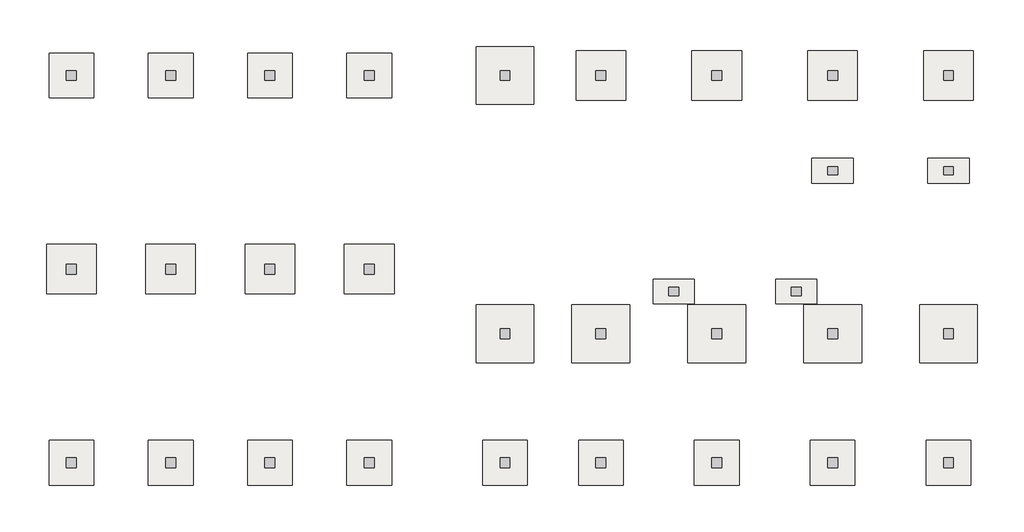
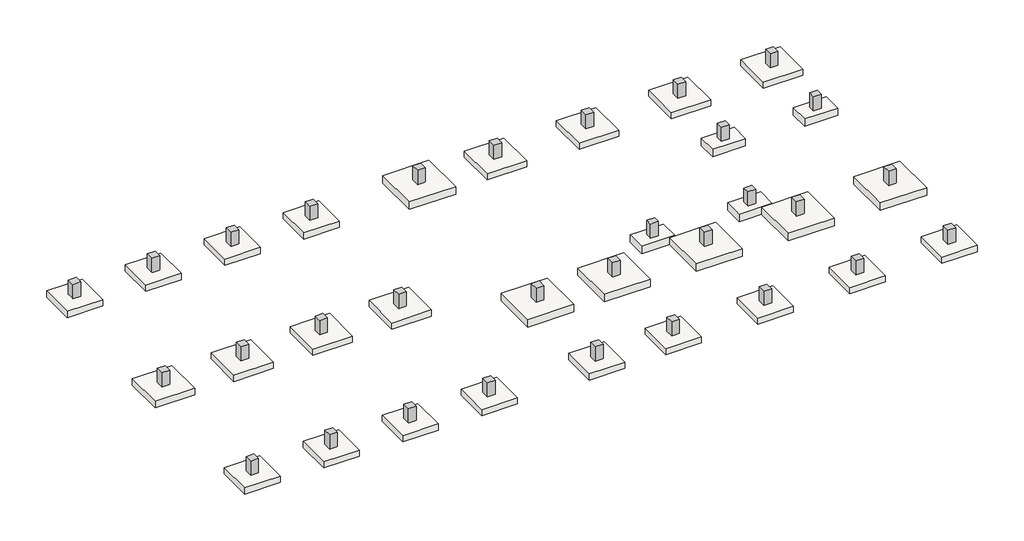
# Not in any storey: 31 columns, 31 slabs.
"""IFC4 building model written with IfcOpenShell, lengths in millimetres."""

from ifc_helpers import new_model, si_unit, frame, origin, place, context, project, spatial, polyline, outline, extrude, faceted_brep, element, save

model = new_model("IFC4")

# Units and contexts
model_context = context("Model", 3, world=origin())
ifc_project = project(units=[si_unit("LENGTHUNIT", "METRE", prefix="MILLI")], contexts=[model_context])

# Site, building
site = spatial("IfcSite", under=ifc_project)
building = spatial("IfcBuilding", under=site)

# Columns
placement = place(None, origin())
element("IfcColumn", 1, ObjectType="RC_Column_Rectangular : H_SC_AR_S15_UG PED_W600xL600_Bit_Anchor", at=placement, inside=building, context=model_context, shape_type="Brep", body=[
    faceted_brep([(300.0, 12499.5208589, -1000.0381366), (300.0, 11899.5208589, -1000.0381366), (-300.0, 11899.5208589, -1000.0381366), (-300.0, 12499.5208589, -1000.0381366), (300.0, 12499.5208589, 149.9618634), (300.0, 11899.5208589, 149.9618634), (300.0, 11899.5208589, -0.0381366), (300.0, 11899.5208589, -500.0381366), (300.0, 12499.5208589, -500.0381366), (300.0, 12499.5208589, -0.0381366), (-300.0, 11899.5208589, 149.9618634), (-300.0, 11899.5208589, -0.0381366), (-300.0, 11899.5208589, -500.0381366), (-300.0, 12499.5208589, 149.9618634), (-300.0, 12499.5208589, -0.0381366), (-300.0, 12499.5208589, -500.0381366)], [[[0, 1, 2, 3]], [[4, 5, 6, 7, 1, 0, 8, 9]], [[5, 10, 11, 12, 2, 1, 7, 6]], [[10, 13, 14, 15, 3, 2, 12, 11]], [[13, 4, 9, 8, 0, 3, 15, 14]], [[4, 13, 10, 5]]]),
])
element("IfcColumn", 2, ObjectType="RC_Column_Rectangular : H_SC_AR_S15_UG PED_W600xL600_Bit_Anchor", at=placement, inside=building, context=model_context, shape_type="SweptSolid", body=[
    extrude(outline(polyline([(6300.0, 12499.5208589), (6300.0, 11899.5208589), (5700.0, 11899.5208589), (5700.0, 12499.5208589), (6300.0, 12499.5208589)])), frame((0.0, 0.0, -1000.0381366), z_axis=(0.0, 0.0, 1.0), x_axis=(1.0, 0.0, 0.0)), (0.0, 0.0, 1.0), 1150.0),
])
element("IfcColumn", 3, ObjectType="RC_Column_Rectangular : H_SC_AR_S15_UG PED_W600xL600_Bit_Anchor", at=placement, inside=building, context=model_context, shape_type="SweptSolid", body=[
    extrude(outline(polyline([(12300.0, 12499.5208589), (12300.0, 11899.5208589), (11700.0, 11899.5208589), (11700.0, 12499.5208589), (12300.0, 12499.5208589)])), frame((0.0, 0.0, -1000.0381366), z_axis=(0.0, 0.0, 1.0), x_axis=(1.0, 0.0, 0.0)), (0.0, 0.0, 1.0), 1150.0),
])
element("IfcColumn", 4, ObjectType="RC_Column_Rectangular : H_SC_AR_S15_UG PED_W600xL600_Bit_Anchor", at=placement, inside=building, context=model_context, shape_type="SweptSolid", body=[
    extrude(outline(polyline([(18300.0, 12499.5208589), (18300.0, 11899.5208589), (17700.0, 11899.5208589), (17700.0, 12499.5208589), (18300.0, 12499.5208589)])), frame((0.0, 0.0, -1000.0381366), z_axis=(0.0, 0.0, 1.0), x_axis=(1.0, 0.0, 0.0)), (0.0, 0.0, 1.0), 1150.0),
])
element("IfcColumn", 5, ObjectType="RC_Column_Rectangular : H_SC_AR_S15_UG PED_W600xL600_Bit_Anchor", at=placement, inside=building, context=model_context, shape_type="Brep", body=[
    faceted_brep([(300.0, 24199.5208589, -1000.0381366), (300.0, 23599.5208589, -1000.0381366), (-300.0, 23599.5208589, -1000.0381366), (-300.0, 24199.5208589, -1000.0381366), (300.0, 24199.5208589, 149.9618634), (300.0, 23599.5208589, 149.9618634), (300.0, 23599.5208589, -0.0381366), (300.0, 23599.5208589, -500.0381366), (300.0, 24199.5208589, -500.0381366), (300.0, 24199.5208589, -0.0381366), (-300.0, 23599.5208589, 149.9618634), (-300.0, 23599.5208589, -0.0381366), (-300.0, 23599.5208589, -500.0381366), (-300.0, 24199.5208589, 149.9618634)], [[[0, 1, 2, 3]], [[4, 5, 6, 7, 1, 0, 8, 9]], [[5, 10, 11, 12, 2, 1, 7, 6]], [[10, 13, 3, 2, 12, 11]], [[13, 4, 9, 8, 0, 3]], [[4, 13, 10, 5]]]),
])
element("IfcColumn", 6, ObjectType="RC_Column_Rectangular : H_SC_AR_S15_UG PED_W600xL600_Bit_Anchor", at=placement, inside=building, context=model_context, shape_type="Brep", body=[
    faceted_brep([(6300.0, 24199.5208589, -1000.0381366), (6300.0, 23599.5208589, -1000.0381366), (5700.0, 23599.5208589, -1000.0381366), (5700.0, 24199.5208589, -1000.0381366), (6300.0, 24199.5208589, 149.9618634), (6300.0, 23599.5208589, 149.9618634), (6300.0, 23599.5208589, -0.0381366), (6300.0, 23599.5208589, -500.0381366), (6300.0, 24199.5208589, -500.0381366), (6300.0, 24199.5208589, -0.0381366), (5700.0, 23599.5208589, 149.9618634), (5700.0, 23599.5208589, -0.0381366), (5700.0, 23599.5208589, -500.0381366), (5700.0, 24199.5208589, 149.9618634), (5700.0, 24199.5208589, -0.0381366), (5700.0, 24199.5208589, -500.0381366)], [[[0, 1, 2, 3]], [[4, 5, 6, 7, 1, 0, 8, 9]], [[5, 10, 11, 12, 2, 1, 7, 6]], [[10, 13, 14, 15, 3, 2, 12, 11]], [[13, 4, 9, 8, 0, 3, 15, 14]], [[4, 13, 10, 5]]]),
])
element("IfcColumn", 7, ObjectType="RC_Column_Rectangular : H_SC_AR_S15_UG PED_W600xL600_Bit_Anchor", at=placement, inside=building, context=model_context, shape_type="Brep", body=[
    faceted_brep([(12300.0, 24199.5208589, -1000.0381366), (12300.0, 23599.5208589, -1000.0381366), (11700.0, 23599.5208589, -1000.0381366), (11700.0, 24199.5208589, -1000.0381366), (12300.0, 24199.5208589, 149.9618634), (12300.0, 23599.5208589, 149.9618634), (12300.0, 23599.5208589, -0.0381366), (12300.0, 23599.5208589, -500.0381366), (12300.0, 24199.5208589, -500.0381366), (12300.0, 24199.5208589, -0.0381366), (11700.0, 23599.5208589, 149.9618634), (11700.0, 23599.5208589, -0.0381366), (11700.0, 23599.5208589, -500.0381366), (11700.0, 24199.5208589, 149.9618634), (11700.0, 24199.5208589, -0.0381366), (11700.0, 24199.5208589, -500.0381366)], [[[0, 1, 2, 3]], [[4, 5, 6, 7, 1, 0, 8, 9]], [[5, 10, 11, 12, 2, 1, 7, 6]], [[10, 13, 14, 15, 3, 2, 12, 11]], [[13, 4, 9, 8, 0, 3, 15, 14]], [[4, 13, 10, 5]]]),
])
element("IfcColumn", 8, ObjectType="RC_Column_Rectangular : H_SC_AR_S15_UG PED_W600xL600_Bit_Anchor", at=placement, inside=building, context=model_context, shape_type="Brep", body=[
    faceted_brep([(18300.0, 24199.5208589, -1000.0381366), (18300.0, 23599.5208589, -1000.0381366), (17700.0, 23599.5208589, -1000.0381366), (17700.0, 24199.5208589, -1000.0381366), (18300.0, 24199.5208589, 149.9618634), (18300.0, 23599.5208589, 149.9618634), (18300.0, 23599.5208589, -0.0381366), (18300.0, 23599.5208589, -500.0381366), (18300.0, 24199.5208589, -500.0381366), (18300.0, 24199.5208589, -0.0381366), (17700.0, 23599.5208589, 149.9618634), (17700.0, 23599.5208589, -0.0381366), (17700.0, 23599.5208589, -500.0381366), (17700.0, 24199.5208589, 149.9618634), (17700.0, 24199.5208589, -0.0381366), (17700.0, 24199.5208589, -500.0381366)], [[[0, 1, 2, 3]], [[4, 5, 6, 7, 1, 0, 8, 9]], [[5, 10, 11, 12, 2, 1, 7, 6]], [[10, 13, 14, 15, 3, 2, 12, 11]], [[13, 4, 9, 8, 0, 3, 15, 14]], [[4, 13, 10, 5]]]),
])
element("IfcColumn", 9, ObjectType="RC_Column_Rectangular : H_SC_AR_S15_UG PED_W600xL600_Bit_Anchor", at=placement, inside=building, context=model_context, shape_type="Brep", body=[
    faceted_brep([(26500.0, 24199.5208589, -1000.0381366), (26500.0, 23599.5208589, -1000.0381366), (25900.0, 23599.5208589, -1000.0381366), (25900.0, 24199.5208589, -1000.0381366), (26500.0, 24199.5208589, 149.9618634), (26500.0, 23599.5208589, 149.9618634), (26500.0, 23599.5208589, -0.0381366), (26500.0, 23599.5208589, -500.0381366), (26500.0, 24199.5208589, -500.0381366), (26500.0, 24199.5208589, -0.0381366), (25900.0, 23599.5208589, 149.9618634), (25900.0, 23599.5208589, -0.0381366), (25900.0, 23599.5208589, -500.0381366), (25900.0, 24199.5208589, 149.9618634), (25900.0, 24199.5208589, -0.0381366), (25900.0, 24199.5208589, -500.0381366)], [[[0, 1, 2, 3]], [[4, 5, 6, 7, 1, 0, 8, 9]], [[5, 10, 11, 12, 2, 1, 7, 6]], [[10, 13, 14, 15, 3, 2, 12, 11]], [[13, 4, 9, 8, 0, 3, 15, 14]], [[4, 13, 10, 5]]]),
])
element("IfcColumn", 10, ObjectType="RC_Column_Rectangular : H_SC_AR_S15_UG PED_W600xL600_Bit_Anchor", at=placement, inside=building, context=model_context, shape_type="Brep", body=[
    faceted_brep([(32300.0, 24199.5208589, -1000.0381366), (32300.0, 23599.5208589, -1000.0381366), (31700.0, 23599.5208589, -1000.0381366), (31700.0, 24199.5208589, -1000.0381366), (32300.0, 24199.5208589, 149.9618634), (32300.0, 23599.5208589, 149.9618634), (32300.0, 23599.5208589, -0.0381366), (32300.0, 23599.5208589, -500.0381366), (32300.0, 24199.5208589, -500.0381366), (32300.0, 24199.5208589, -0.0381366), (31700.0, 23599.5208589, 149.9618634), (31700.0, 23599.5208589, -0.0381366), (31700.0, 23599.5208589, -500.0381366), (31700.0, 24199.5208589, 149.9618634), (31700.0, 24199.5208589, -0.0381366), (31700.0, 24199.5208589, -500.0381366)], [[[0, 1, 2, 3]], [[4, 5, 6, 7, 1, 0, 8, 9]], [[5, 10, 11, 12, 2, 1, 7, 6]], [[10, 13, 14, 15, 3, 2, 12, 11]], [[13, 4, 9, 8, 0, 3, 15, 14]], [[4, 13, 10, 5]]]),
])
element("IfcColumn", 11, ObjectType="RC_Column_Rectangular : H_SC_AR_S15_UG PED_W600xL600_Bit_Anchor", at=placement, inside=building, context=model_context, shape_type="Brep", body=[
    faceted_brep([(39300.0, 24199.5208589, -1000.0381366), (39300.0, 23599.5208589, -1000.0381366), (38700.0, 23599.5208589, -1000.0381366), (38700.0, 24199.5208589, -1000.0381366), (39300.0, 24199.5208589, 149.9618634), (39300.0, 23599.5208589, 149.9618634), (39300.0, 23599.5208589, -0.0381366), (39300.0, 23599.5208589, -500.0381366), (39300.0, 24199.5208589, -500.0381366), (39300.0, 24199.5208589, -0.0381366), (38700.0, 23599.5208589, 149.9618634), (38700.0, 23599.5208589, -0.0381366), (38700.0, 23599.5208589, -500.0381366), (38700.0, 24199.5208589, 149.9618634), (38700.0, 24199.5208589, -0.0381366), (38700.0, 24199.5208589, -500.0381366)], [[[0, 1, 2, 3]], [[4, 5, 6, 7, 1, 0, 8, 9]], [[5, 10, 11, 12, 2, 1, 7, 6]], [[10, 13, 14, 15, 3, 2, 12, 11]], [[13, 4, 9, 8, 0, 3, 15, 14]], [[4, 13, 10, 5]]]),
])
element("IfcColumn", 12, ObjectType="RC_Column_Rectangular : H_SC_AR_S15_UG PED_W600xL600_Bit_Anchor", at=placement, inside=building, context=model_context, shape_type="Brep", body=[
    faceted_brep([(46300.0, 24199.5208589, -1000.0381366), (46300.0, 23599.5208589, -1000.0381366), (45700.0, 23599.5208589, -1000.0381366), (45700.0, 24199.5208589, -1000.0381366), (46300.0, 24199.5208589, 149.9618634), (46300.0, 23599.5208589, 149.9618634), (46300.0, 23599.5208589, -0.0381366), (46300.0, 23599.5208589, -500.0381366), (46300.0, 24199.5208589, -500.0381366), (46300.0, 24199.5208589, -0.0381366), (45700.0, 23599.5208589, 149.9618634), (45700.0, 23599.5208589, -0.0381366), (45700.0, 23599.5208589, -500.0381366), (45700.0, 24199.5208589, 149.9618634), (45700.0, 24199.5208589, -0.0381366), (45700.0, 24199.5208589, -500.0381366)], [[[0, 1, 2, 3]], [[4, 5, 6, 7, 1, 0, 8, 9]], [[5, 10, 11, 12, 2, 1, 7, 6]], [[10, 13, 14, 15, 3, 2, 12, 11]], [[13, 4, 9, 8, 0, 3, 15, 14]], [[4, 13, 10, 5]]]),
])
element("IfcColumn", 13, ObjectType="RC_Column_Rectangular : H_SC_AR_S15_UG PED_W600xL600_Bit_Anchor", at=placement, inside=building, context=model_context, shape_type="Brep", body=[
    faceted_brep([(53300.0, 24199.5208589, -1000.0381366), (53300.0, 23599.5208589, -1000.0381366), (52700.0, 23599.5208589, -1000.0381366), (52700.0, 24199.5208589, -1000.0381366), (53300.0, 24199.5208589, 149.9618634), (53300.0, 23599.5208589, 149.9618634), (53300.0, 23599.5208589, -0.0381366), (53300.0, 23599.5208589, -500.0381366), (52700.0, 23599.5208589, 149.9618634), (52700.0, 23599.5208589, -0.0381366), (52700.0, 23599.5208589, -500.0381366), (52700.0, 24199.5208589, 149.9618634), (52700.0, 24199.5208589, -0.0381366), (52700.0, 24199.5208589, -500.0381366)], [[[0, 1, 2, 3]], [[4, 5, 6, 7, 1, 0]], [[5, 8, 9, 10, 2, 1, 7, 6]], [[8, 11, 12, 13, 3, 2, 10, 9]], [[11, 4, 0, 3, 13, 12]], [[4, 11, 8, 5]]]),
])
element("IfcColumn", 14, ObjectType="RC_Column_Rectangular : H_SC_AR_S15_UG PED_W600xL600_Bit_Anchor", at=placement, inside=building, context=model_context, shape_type="SweptSolid", body=[
    extrude(outline(polyline([(26500.0, 8599.5208589), (26500.0, 7999.5208589), (25900.0, 7999.5208589), (25900.0, 8599.5208589), (26500.0, 8599.5208589)])), frame((0.0, 0.0, -1000.0381366), z_axis=(0.0, 0.0, 1.0), x_axis=(1.0, 0.0, 0.0)), (0.0, 0.0, 1.0), 1150.0),
])
element("IfcColumn", 15, ObjectType="RC_Column_Rectangular : H_SC_AR_S15_UG PED_W600xL600_Bit_Anchor", at=placement, inside=building, context=model_context, shape_type="SweptSolid", body=[
    extrude(outline(polyline([(32300.0, 8599.5208589), (32300.0, 7999.5208589), (31700.0, 7999.5208589), (31700.0, 8599.5208589), (32300.0, 8599.5208589)])), frame((0.0, 0.0, -1000.0381366), z_axis=(0.0, 0.0, 1.0), x_axis=(1.0, 0.0, 0.0)), (0.0, 0.0, 1.0), 1150.0),
])
element("IfcColumn", 16, ObjectType="RC_Column_Rectangular : H_SC_AR_S15_UG PED_W600xL600_Bit_Anchor", at=placement, inside=building, context=model_context, shape_type="SweptSolid", body=[
    extrude(outline(polyline([(39300.0, 8599.5208589), (39300.0, 7999.5208589), (38700.0, 7999.5208589), (38700.0, 8599.5208589), (39300.0, 8599.5208589)])), frame((0.0, 0.0, -1000.0381366), z_axis=(0.0, 0.0, 1.0), x_axis=(1.0, 0.0, 0.0)), (0.0, 0.0, 1.0), 1150.0),
])
element("IfcColumn", 17, ObjectType="RC_Column_Rectangular : H_SC_AR_S15_UG PED_W600xL600_Bit_Anchor", at=placement, inside=building, context=model_context, shape_type="SweptSolid", body=[
    extrude(outline(polyline([(46300.0, 8599.5208589), (46300.0, 7999.5208589), (45700.0, 7999.5208589), (45700.0, 8599.5208589), (46300.0, 8599.5208589)])), frame((0.0, 0.0, -1000.0381366), z_axis=(0.0, 0.0, 1.0), x_axis=(1.0, 0.0, 0.0)), (0.0, 0.0, 1.0), 1150.0),
])
element("IfcColumn", 18, ObjectType="RC_Column_Rectangular : H_SC_AR_S15_UG PED_W600xL600_Bit_Anchor", at=placement, inside=building, context=model_context, shape_type="Brep", body=[
    faceted_brep([(53300.0, 8599.5208589, -1000.0381366), (53300.0, 7999.5208589, -1000.0381366), (52700.0, 7999.5208589, -1000.0381366), (52700.0, 8599.5208589, -1000.0381366), (53300.0, 8599.5208589, 149.9618634), (53300.0, 7999.5208589, 149.9618634), (53300.0, 7999.5208589, -0.0381366), (53300.0, 7999.5208589, -500.0381366), (53300.0, 8599.5208589, -500.0381366), (53300.0, 8599.5208589, -0.0381366), (52700.0, 7999.5208589, 149.9618634), (52700.0, 7999.5208589, -0.0381366), (52700.0, 7999.5208589, -500.0381366), (52700.0, 8599.5208589, 149.9618634), (52700.0, 8599.5208589, -0.0381366), (52700.0, 8599.5208589, -500.0381366)], [[[0, 1, 2, 3]], [[4, 5, 6, 7, 1, 0, 8, 9]], [[5, 10, 11, 12, 2, 1, 7, 6]], [[10, 13, 14, 15, 3, 2, 12, 11]], [[13, 4, 9, 8, 0, 3, 15, 14]], [[4, 13, 10, 5]]]),
])
element("IfcColumn", 19, ObjectType="RC_Column_Rectangular : H_SC_AR_S15_UG PED_W600xL600_Bit_Anchor", at=placement, inside=building, context=model_context, shape_type="Brep", body=[
    faceted_brep([(300.0, 799.5208589, -1000.0381366), (300.0, 199.5208589, -1000.0381366), (-300.0, 199.5208589, -1000.0381366), (-300.0, 799.5208589, -1000.0381366), (300.0, 799.5208589, 149.9618634), (300.0, 199.5208589, 149.9618634), (300.0, 199.5208589, -0.0381366), (300.0, 199.5208589, -500.0381366), (300.0, 799.5208589, -500.0381366), (300.0, 799.5208589, -0.0381366), (-300.0, 199.5208589, 149.9618634), (-300.0, 799.5208589, 149.9618634), (-300.0, 799.5208589, -0.0381366), (-300.0, 799.5208589, -500.0381366)], [[[0, 1, 2, 3]], [[4, 5, 6, 7, 1, 0, 8, 9]], [[5, 10, 2, 1, 7, 6]], [[10, 11, 12, 13, 3, 2]], [[11, 4, 9, 8, 0, 3, 13, 12]], [[4, 11, 10, 5]]]),
])
element("IfcColumn", 20, ObjectType="RC_Column_Rectangular : H_SC_AR_S15_UG PED_W600xL600_Bit_Anchor", at=placement, inside=building, context=model_context, shape_type="Brep", body=[
    faceted_brep([(6300.0, 799.5208589, -1000.0381366), (6300.0, 199.5208589, -1000.0381366), (5700.0, 199.5208589, -1000.0381366), (5700.0, 799.5208589, -1000.0381366), (6300.0, 799.5208589, 149.9618634), (6300.0, 199.5208589, 149.9618634), (6300.0, 199.5208589, -0.0381366), (6300.0, 199.5208589, -500.0381366), (6300.0, 799.5208589, -500.0381366), (6300.0, 799.5208589, -0.0381366), (5700.0, 199.5208589, 149.9618634), (5700.0, 199.5208589, -0.0381366), (5700.0, 199.5208589, -500.0381366), (5700.0, 799.5208589, 149.9618634), (5700.0, 799.5208589, -0.0381366), (5700.0, 799.5208589, -500.0381366)], [[[0, 1, 2, 3]], [[4, 5, 6, 7, 1, 0, 8, 9]], [[5, 10, 11, 12, 2, 1, 7, 6]], [[10, 13, 14, 15, 3, 2, 12, 11]], [[13, 4, 9, 8, 0, 3, 15, 14]], [[4, 13, 10, 5]]]),
])
element("IfcColumn", 21, ObjectType="RC_Column_Rectangular : H_SC_AR_S15_UG PED_W600xL600_Bit_Anchor", at=placement, inside=building, context=model_context, shape_type="Brep", body=[
    faceted_brep([(12300.0, 799.5208589, -1000.0381366), (12300.0, 199.5208589, -1000.0381366), (11700.0, 199.5208589, -1000.0381366), (11700.0, 799.5208589, -1000.0381366), (12300.0, 799.5208589, 149.9618634), (12300.0, 199.5208589, 149.9618634), (12300.0, 199.5208589, -0.0381366), (12300.0, 199.5208589, -500.0381366), (12300.0, 799.5208589, -500.0381366), (12300.0, 799.5208589, -0.0381366), (11700.0, 199.5208589, 149.9618634), (11700.0, 199.5208589, -0.0381366), (11700.0, 199.5208589, -500.0381366), (11700.0, 799.5208589, 149.9618634), (11700.0, 799.5208589, -0.0381366), (11700.0, 799.5208589, -500.0381366)], [[[0, 1, 2, 3]], [[4, 5, 6, 7, 1, 0, 8, 9]], [[5, 10, 11, 12, 2, 1, 7, 6]], [[10, 13, 14, 15, 3, 2, 12, 11]], [[13, 4, 9, 8, 0, 3, 15, 14]], [[4, 13, 10, 5]]]),
])
element("IfcColumn", 22, ObjectType="RC_Column_Rectangular : H_SC_AR_S15_UG PED_W600xL600_Bit_Anchor", at=placement, inside=building, context=model_context, shape_type="Brep", body=[
    faceted_brep([(18300.0, 799.5208589, -1000.0381366), (18300.0, 199.5208589, -1000.0381366), (17700.0, 199.5208589, -1000.0381366), (17700.0, 799.5208589, -1000.0381366), (18300.0, 799.5208589, 149.9618634), (18300.0, 199.5208589, 149.9618634), (18300.0, 199.5208589, -0.0381366), (18300.0, 199.5208589, -500.0381366), (18300.0, 799.5208589, -500.0381366), (18300.0, 799.5208589, -0.0381366), (17700.0, 199.5208589, 149.9618634), (17700.0, 199.5208589, -0.0381366), (17700.0, 199.5208589, -500.0381366), (17700.0, 799.5208589, 149.9618634), (17700.0, 799.5208589, -0.0381366), (17700.0, 799.5208589, -500.0381366)], [[[0, 1, 2, 3]], [[4, 5, 6, 7, 1, 0, 8, 9]], [[5, 10, 11, 12, 2, 1, 7, 6]], [[10, 13, 14, 15, 3, 2, 12, 11]], [[13, 4, 9, 8, 0, 3, 15, 14]], [[4, 13, 10, 5]]]),
])
element("IfcColumn", 23, ObjectType="RC_Column_Rectangular : H_SC_AR_S15_UG PED_W600xL600_Bit_Anchor", at=placement, inside=building, context=model_context, shape_type="Brep", body=[
    faceted_brep([(26500.0, 799.5208589, -1000.0381366), (26500.0, 199.5208589, -1000.0381366), (25900.0, 199.5208589, -1000.0381366), (25900.0, 799.5208589, -1000.0381366), (26500.0, 799.5208589, 149.9618634), (26500.0, 199.5208589, 149.9618634), (26500.0, 199.5208589, -0.0381366), (26500.0, 199.5208589, -500.0381366), (26500.0, 799.5208589, -500.0381366), (26500.0, 799.5208589, -0.0381366), (25900.0, 199.5208589, 149.9618634), (25900.0, 199.5208589, -0.0381366), (25900.0, 199.5208589, -500.0381366), (25900.0, 799.5208589, 149.9618634), (25900.0, 799.5208589, -0.0381366), (25900.0, 799.5208589, -500.0381366)], [[[0, 1, 2, 3]], [[4, 5, 6, 7, 1, 0, 8, 9]], [[5, 10, 11, 12, 2, 1, 7, 6]], [[10, 13, 14, 15, 3, 2, 12, 11]], [[13, 4, 9, 8, 0, 3, 15, 14]], [[4, 13, 10, 5]]]),
])
element("IfcColumn", 24, ObjectType="RC_Column_Rectangular : H_SC_AR_S15_UG PED_W600xL600_Bit_Anchor", at=placement, inside=building, context=model_context, shape_type="Brep", body=[
    faceted_brep([(32300.0, 799.5208589, -1000.0381366), (32300.0, 199.5208589, -1000.0381366), (31700.0, 199.5208589, -1000.0381366), (31700.0, 799.5208589, -1000.0381366), (32300.0, 799.5208589, 149.9618634), (32300.0, 199.5208589, 149.9618634), (32300.0, 199.5208589, -0.0381366), (32300.0, 199.5208589, -500.0381366), (32300.0, 799.5208589, -500.0381366), (32300.0, 799.5208589, -0.0381366), (31700.0, 199.5208589, 149.9618634), (31700.0, 199.5208589, -0.0381366), (31700.0, 199.5208589, -500.0381366), (31700.0, 799.5208589, 149.9618634), (31700.0, 799.5208589, -0.0381366), (31700.0, 799.5208589, -500.0381366)], [[[0, 1, 2, 3]], [[4, 5, 6, 7, 1, 0, 8, 9]], [[5, 10, 11, 12, 2, 1, 7, 6]], [[10, 13, 14, 15, 3, 2, 12, 11]], [[13, 4, 9, 8, 0, 3, 15, 14]], [[4, 13, 10, 5]]]),
])
element("IfcColumn", 25, ObjectType="RC_Column_Rectangular : H_SC_AR_S15_UG PED_W600xL600_Bit_Anchor", at=placement, inside=building, context=model_context, shape_type="Brep", body=[
    faceted_brep([(39300.0, 799.5208589, -1000.0381366), (39300.0, 199.5208589, -1000.0381366), (38700.0, 199.5208589, -1000.0381366), (38700.0, 799.5208589, -1000.0381366), (39300.0, 799.5208589, 149.9618634), (39300.0, 199.5208589, 149.9618634), (39300.0, 199.5208589, -0.0381366), (39300.0, 199.5208589, -500.0381366), (39300.0, 799.5208589, -500.0381366), (39300.0, 799.5208589, -0.0381366), (38700.0, 199.5208589, 149.9618634), (38700.0, 199.5208589, -0.0381366), (38700.0, 199.5208589, -500.0381366), (38700.0, 799.5208589, 149.9618634), (38700.0, 799.5208589, -0.0381366), (38700.0, 799.5208589, -500.0381366)], [[[0, 1, 2, 3]], [[4, 5, 6, 7, 1, 0, 8, 9]], [[5, 10, 11, 12, 2, 1, 7, 6]], [[10, 13, 14, 15, 3, 2, 12, 11]], [[13, 4, 9, 8, 0, 3, 15, 14]], [[4, 13, 10, 5]]]),
])
element("IfcColumn", 26, ObjectType="RC_Column_Rectangular : H_SC_AR_S15_UG PED_W600xL600_Bit_Anchor", at=placement, inside=building, context=model_context, shape_type="Brep", body=[
    faceted_brep([(46300.0, 799.5208589, -1000.0381366), (46300.0, 199.5208589, -1000.0381366), (45700.0, 199.5208589, -1000.0381366), (45700.0, 799.5208589, -1000.0381366), (46300.0, 799.5208589, 149.9618634), (46300.0, 199.5208589, 149.9618634), (46300.0, 199.5208589, -0.0381366), (46300.0, 199.5208589, -500.0381366), (46300.0, 799.5208589, -500.0381366), (46300.0, 799.5208589, -0.0381366), (45700.0, 199.5208589, 149.9618634), (45700.0, 199.5208589, -0.0381366), (45700.0, 199.5208589, -500.0381366), (45700.0, 799.5208589, 149.9618634), (45700.0, 799.5208589, -0.0381366), (45700.0, 799.5208589, -500.0381366)], [[[0, 1, 2, 3]], [[4, 5, 6, 7, 1, 0, 8, 9]], [[5, 10, 11, 12, 2, 1, 7, 6]], [[10, 13, 14, 15, 3, 2, 12, 11]], [[13, 4, 9, 8, 0, 3, 15, 14]], [[4, 13, 10, 5]]]),
])
element("IfcColumn", 27, ObjectType="RC_Column_Rectangular : H_SC_AR_S15_UG PED_W600xL600_Bit_Anchor", at=placement, inside=building, context=model_context, shape_type="Brep", body=[
    faceted_brep([(53300.0, 799.5208589, -1000.0381366), (53300.0, 199.5208589, -1000.0381366), (52700.0, 199.5208589, -1000.0381366), (52700.0, 799.5208589, -1000.0381366), (53300.0, 799.5208589, 149.9618634), (53300.0, 199.5208589, 149.9618634), (53300.0, 799.5208589, -500.0381366), (53300.0, 799.5208589, -0.0381366), (52700.0, 199.5208589, 149.9618634), (52700.0, 199.5208589, -0.0381366), (52700.0, 199.5208589, -500.0381366), (52700.0, 799.5208589, 149.9618634), (52700.0, 799.5208589, -0.0381366), (52700.0, 799.5208589, -500.0381366)], [[[0, 1, 2, 3]], [[4, 5, 1, 0, 6, 7]], [[5, 8, 9, 10, 2, 1]], [[8, 11, 12, 13, 3, 2, 10, 9]], [[11, 4, 7, 6, 0, 3, 13, 12]], [[4, 11, 8, 5]]]),
])
element("IfcColumn", 28, ObjectType="RC_Column_Rectangular : H_SC_AR_S15_UG PED_W600xL500_Bit_PD1A", at=placement, inside=building, context=model_context, shape_type="Brep", body=[
    faceted_brep([(52700.0, 18399.5208589, -1000.0381366), (53300.0, 18399.5208589, -1000.0381366), (53300.0, 17899.5208589, -1000.0381366), (52700.0, 17899.5208589, -1000.0381366), (52700.0, 18399.5208589, 149.9618634), (53300.0, 18399.5208589, 149.9618634), (53300.0, 18399.5208589, -0.0381366), (53300.0, 18399.5208589, -500.0381366), (52700.0, 18399.5208589, -500.0381366), (52700.0, 18399.5208589, -0.0381366), (53300.0, 17899.5208589, 149.9618634), (53300.0, 17899.5208589, -0.0381366), (53300.0, 17899.5208589, -500.0381366), (52700.0, 17899.5208589, 149.9618634), (52700.0, 17899.5208589, -0.0381366), (52700.0, 17899.5208589, -500.0381366)], [[[0, 1, 2, 3]], [[4, 5, 6, 7, 1, 0, 8, 9]], [[5, 10, 11, 12, 2, 1, 7, 6]], [[10, 13, 14, 15, 3, 2, 12, 11]], [[13, 4, 9, 8, 0, 3, 15, 14]], [[4, 13, 10, 5]]]),
])
element("IfcColumn", 29, ObjectType="RC_Column_Rectangular : H_SC_AR_S15_UG PED_W600xL500_Bit_PD1A", at=placement, inside=building, context=model_context, shape_type="SweptSolid", body=[
    extrude(outline(polyline([(45700.0, 18399.5208589), (46300.0, 18399.5208589), (46300.0, 17899.5208589), (45700.0, 17899.5208589), (45700.0, 18399.5208589)])), frame((0.0, 0.0, -1000.0381366), z_axis=(0.0, 0.0, 1.0), x_axis=(1.0, 0.0, 0.0)), (0.0, 0.0, 1.0), 1150.0),
])
element("IfcColumn", 30, ObjectType="RC_Column_Rectangular : H_SC_AR_S15_UG PED_W600xL500_Bit_PD1A", at=placement, inside=building, context=model_context, shape_type="SweptSolid", body=[
    extrude(outline(polyline([(36100.0, 11099.5208589), (36700.0, 11099.5208589), (36700.0, 10599.5208589), (36100.0, 10599.5208589), (36100.0, 11099.5208589)])), frame((0.0, 0.0, -1000.0381366), z_axis=(0.0, 0.0, 1.0), x_axis=(1.0, 0.0, 0.0)), (0.0, 0.0, 1.0), 1150.0),
])
element("IfcColumn", 31, ObjectType="RC_Column_Rectangular : H_SC_AR_S15_UG PED_W600xL500_Bit_PD1A", at=placement, inside=building, context=model_context, shape_type="SweptSolid", body=[
    extrude(outline(polyline([(43500.0, 11099.5208589), (44100.0, 11099.5208589), (44100.0, 10599.5208589), (43500.0, 10599.5208589), (43500.0, 11099.5208589)])), frame((0.0, 0.0, -1000.0381366), z_axis=(0.0, 0.0, 1.0), x_axis=(1.0, 0.0, 0.0)), (0.0, 0.0, 1.0), 1150.0),
])

# Slabs
element("IfcSlab", 32, ObjectType="Foundation Rectangular (Non-Pile) : H_SF_AR_S18_W3000xL3000xT500_Bitumen_F2", at=placement, inside=building, context=model_context, shape_type="SweptSolid", body=[
    extrude(outline(polyline([(1500.0, 13699.5208589), (1500.0, 10699.5208589), (-1500.0, 10699.5208589), (-1500.0, 13699.5208589), (1500.0, 13699.5208589)])), frame((0.0, 0.0, -1500.0381366), z_axis=(0.0, 0.0, 1.0), x_axis=(1.0, 0.0, 0.0)), (0.0, 0.0, 1.0), 500.0),
])
element("IfcSlab", 33, ObjectType="Foundation Rectangular (Non-Pile) : H_SF_AR_S18_W3000xL3000xT500_Bitumen_F2", at=placement, inside=building, context=model_context, shape_type="SweptSolid", body=[
    extrude(outline(polyline([(7500.0, 13699.5208589), (7500.0, 10699.5208589), (4500.0, 10699.5208589), (4500.0, 13699.5208589), (7500.0, 13699.5208589)])), frame((0.0, 0.0, -1500.0381366), z_axis=(0.0, 0.0, 1.0), x_axis=(1.0, 0.0, 0.0)), (0.0, 0.0, 1.0), 500.0),
])
element("IfcSlab", 34, ObjectType="Foundation Rectangular (Non-Pile) : H_SF_AR_S18_W3000xL3000xT500_Bitumen_F2", at=placement, inside=building, context=model_context, shape_type="SweptSolid", body=[
    extrude(outline(polyline([(13500.0, 13699.5208589), (13500.0, 10699.5208589), (10500.0, 10699.5208589), (10500.0, 13699.5208589), (13500.0, 13699.5208589)])), frame((0.0, 0.0, -1500.0381366), z_axis=(0.0, 0.0, 1.0), x_axis=(1.0, 0.0, 0.0)), (0.0, 0.0, 1.0), 500.0),
])
element("IfcSlab", 35, ObjectType="Foundation Rectangular (Non-Pile) : H_SF_AR_S18_W3000xL3000xT500_Bitumen_F2", at=placement, inside=building, context=model_context, shape_type="SweptSolid", body=[
    extrude(outline(polyline([(19500.0, 13699.5208589), (19500.0, 10699.5208589), (16500.0, 10699.5208589), (16500.0, 13699.5208589), (19500.0, 13699.5208589)])), frame((0.0, 0.0, -1500.0381366), z_axis=(0.0, 0.0, 1.0), x_axis=(1.0, 0.0, 0.0)), (0.0, 0.0, 1.0), 500.0),
])
element("IfcSlab", 36, ObjectType="Foundation Rectangular (Non-Pile) : H_SF_AR_S18_W2700xL2700xT500_Bitumen_F1", at=placement, inside=building, context=model_context, shape_type="SweptSolid", body=[
    extrude(outline(polyline([(1350.0, 25249.5208589), (1350.0, 22549.5208589), (-1350.0, 22549.5208589), (-1350.0, 25249.5208589), (1350.0, 25249.5208589)])), frame((0.0, 0.0, -1500.0381366), z_axis=(0.0, 0.0, 1.0), x_axis=(1.0, 0.0, 0.0)), (0.0, 0.0, 1.0), 500.0),
])
element("IfcSlab", 37, ObjectType="Foundation Rectangular (Non-Pile) : H_SF_AR_S18_W2700xL2700xT500_Bitumen_F1", at=placement, inside=building, context=model_context, shape_type="SweptSolid", body=[
    extrude(outline(polyline([(7350.0, 25249.5208589), (7350.0, 22549.5208589), (4650.0, 22549.5208589), (4650.0, 25249.5208589), (7350.0, 25249.5208589)])), frame((0.0, 0.0, -1500.0381366), z_axis=(0.0, 0.0, 1.0), x_axis=(1.0, 0.0, 0.0)), (0.0, 0.0, 1.0), 500.0),
])
element("IfcSlab", 38, ObjectType="Foundation Rectangular (Non-Pile) : H_SF_AR_S18_W2700xL2700xT500_Bitumen_F1", at=placement, inside=building, context=model_context, shape_type="SweptSolid", body=[
    extrude(outline(polyline([(13350.0, 25249.5208589), (13350.0, 22549.5208589), (10650.0, 22549.5208589), (10650.0, 25249.5208589), (13350.0, 25249.5208589)])), frame((0.0, 0.0, -1500.0381366), z_axis=(0.0, 0.0, 1.0), x_axis=(1.0, 0.0, 0.0)), (0.0, 0.0, 1.0), 500.0),
])
element("IfcSlab", 39, ObjectType="Foundation Rectangular (Non-Pile) : H_SF_AR_S18_W2700xL2700xT500_Bitumen_F1", at=placement, inside=building, context=model_context, shape_type="SweptSolid", body=[
    extrude(outline(polyline([(19350.0, 25249.5208589), (19350.0, 22549.5208589), (16650.0, 22549.5208589), (16650.0, 25249.5208589), (19350.0, 25249.5208589)])), frame((0.0, 0.0, -1500.0381366), z_axis=(0.0, 0.0, 1.0), x_axis=(1.0, 0.0, 0.0)), (0.0, 0.0, 1.0), 500.0),
])
element("IfcSlab", 40, ObjectType="Foundation Rectangular (Non-Pile) : H_SF_AR_S18_W3500xL3500xT600_Bitumen_F3", at=placement, inside=building, context=model_context, shape_type="SweptSolid", body=[
    extrude(outline(polyline([(27950.0, 25649.5208589), (27950.0, 22149.5208589), (24450.0, 22149.5208589), (24450.0, 25649.5208589), (27950.0, 25649.5208589)])), frame((0.0, 0.0, -1600.0381366), z_axis=(0.0, 0.0, 1.0), x_axis=(1.0, 0.0, 0.0)), (0.0, 0.0, 1.0), 600.0),
])
element("IfcSlab", 41, ObjectType="Foundation Rectangular (Non-Pile) : H_SF_AR_S18_W3000xL3000xT500_Bitumen_F2A", at=placement, inside=building, context=model_context, shape_type="SweptSolid", body=[
    extrude(outline(polyline([(33500.0, 25399.5208589), (33500.0, 22399.5208589), (30500.0, 22399.5208589), (30500.0, 25399.5208589), (33500.0, 25399.5208589)])), frame((0.0, 0.0, -1500.0381366), z_axis=(0.0, 0.0, 1.0), x_axis=(1.0, 0.0, 0.0)), (0.0, 0.0, 1.0), 500.0),
])
element("IfcSlab", 42, ObjectType="Foundation Rectangular (Non-Pile) : H_SF_AR_S18_W3000xL3000xT500_Bitumen_F2A", at=placement, inside=building, context=model_context, shape_type="SweptSolid", body=[
    extrude(outline(polyline([(40500.0, 25399.5208589), (40500.0, 22399.5208589), (37500.0, 22399.5208589), (37500.0, 25399.5208589), (40500.0, 25399.5208589)])), frame((0.0, 0.0, -1500.0381366), z_axis=(0.0, 0.0, 1.0), x_axis=(1.0, 0.0, 0.0)), (0.0, 0.0, 1.0), 500.0),
])
element("IfcSlab", 43, ObjectType="Foundation Rectangular (Non-Pile) : H_SF_AR_S18_W3000xL3000xT500_Bitumen_F2A", at=placement, inside=building, context=model_context, shape_type="SweptSolid", body=[
    extrude(outline(polyline([(47500.0, 25399.5208589), (47500.0, 22399.5208589), (44500.0, 22399.5208589), (44500.0, 25399.5208589), (47500.0, 25399.5208589)])), frame((0.0, 0.0, -1500.0381366), z_axis=(0.0, 0.0, 1.0), x_axis=(1.0, 0.0, 0.0)), (0.0, 0.0, 1.0), 500.0),
])
element("IfcSlab", 44, ObjectType="Foundation Rectangular (Non-Pile) : H_SF_AR_S18_W3000xL3000xT500_Bitumen_F2A", at=placement, inside=building, context=model_context, shape_type="SweptSolid", body=[
    extrude(outline(polyline([(54500.0, 25399.5208589), (54500.0, 22399.5208589), (51500.0, 22399.5208589), (51500.0, 25399.5208589), (54500.0, 25399.5208589)])), frame((0.0, 0.0, -1500.0381366), z_axis=(0.0, 0.0, 1.0), x_axis=(1.0, 0.0, 0.0)), (0.0, 0.0, 1.0), 500.0),
])
element("IfcSlab", 45, ObjectType="Foundation Rectangular (Non-Pile) : H_SF_AR_S18_W3500xL3500xT600_Bitumen_F3", at=placement, inside=building, context=model_context, shape_type="SweptSolid", body=[
    extrude(outline(polyline([(27950.0, 10049.5208589), (27950.0, 6549.5208589), (24450.0, 6549.5208589), (24450.0, 10049.5208589), (27950.0, 10049.5208589)])), frame((0.0, 0.0, -1600.0381366), z_axis=(0.0, 0.0, 1.0), x_axis=(1.0, 0.0, 0.0)), (0.0, 0.0, 1.0), 600.0),
])
element("IfcSlab", 46, ObjectType="Foundation Rectangular (Non-Pile) : H_SF_AR_S18_W3500xL3500xT600_Bitumen_F3", at=placement, inside=building, context=model_context, shape_type="SweptSolid", body=[
    extrude(outline(polyline([(33750.0, 10049.5208589), (33750.0, 6549.5208589), (30250.0, 6549.5208589), (30250.0, 10049.5208589), (33750.0, 10049.5208589)])), frame((0.0, 0.0, -1600.0381366), z_axis=(0.0, 0.0, 1.0), x_axis=(1.0, 0.0, 0.0)), (0.0, 0.0, 1.0), 600.0),
])
element("IfcSlab", 47, ObjectType="Foundation Rectangular (Non-Pile) : H_SF_AR_S18_W3500xL3500xT600_Bitumen_F3", at=placement, inside=building, context=model_context, shape_type="SweptSolid", body=[
    extrude(outline(polyline([(40750.0, 10049.5208589), (40750.0, 6549.5208589), (37250.0, 6549.5208589), (37250.0, 10049.5208589), (40750.0, 10049.5208589)])), frame((0.0, 0.0, -1600.0381366), z_axis=(0.0, 0.0, 1.0), x_axis=(1.0, 0.0, 0.0)), (0.0, 0.0, 1.0), 600.0),
])
element("IfcSlab", 48, ObjectType="Foundation Rectangular (Non-Pile) : H_SF_AR_S18_W3500xL3500xT600_Bitumen_F3", at=placement, inside=building, context=model_context, shape_type="SweptSolid", body=[
    extrude(outline(polyline([(47750.0, 10049.5208589), (47750.0, 6549.5208589), (44250.0, 6549.5208589), (44250.0, 10049.5208589), (47750.0, 10049.5208589)])), frame((0.0, 0.0, -1600.0381366), z_axis=(0.0, 0.0, 1.0), x_axis=(1.0, 0.0, 0.0)), (0.0, 0.0, 1.0), 600.0),
])
element("IfcSlab", 49, ObjectType="Foundation Rectangular (Non-Pile) : H_SF_AR_S18_W3500xL3500xT600_Bitumen_F3", at=placement, inside=building, context=model_context, shape_type="SweptSolid", body=[
    extrude(outline(polyline([(54750.0, 10049.5208589), (54750.0, 6549.5208589), (51250.0, 6549.5208589), (51250.0, 10049.5208589), (54750.0, 10049.5208589)])), frame((0.0, 0.0, -1600.0381366), z_axis=(0.0, 0.0, 1.0), x_axis=(1.0, 0.0, 0.0)), (0.0, 0.0, 1.0), 600.0),
])
element("IfcSlab", 50, ObjectType="Foundation Rectangular (Non-Pile) : H_SF_AR_S18_W2700xL2700xT500_Bitumen_F1A", at=placement, inside=building, context=model_context, shape_type="SweptSolid", body=[
    extrude(outline(polyline([(1350.0, 1849.5208589), (1350.0, -850.4791411), (-1350.0, -850.4791411), (-1350.0, 1849.5208589), (1350.0, 1849.5208589)])), frame((0.0, 0.0, -1500.0381366), z_axis=(0.0, 0.0, 1.0), x_axis=(1.0, 0.0, 0.0)), (0.0, 0.0, 1.0), 500.0),
])
element("IfcSlab", 51, ObjectType="Foundation Rectangular (Non-Pile) : H_SF_AR_S18_W2700xL2700xT500_Bitumen_F1", at=placement, inside=building, context=model_context, shape_type="SweptSolid", body=[
    extrude(outline(polyline([(7350.0, 1849.5208589), (7350.0, -850.4791411), (4650.0, -850.4791411), (4650.0, 1849.5208589), (7350.0, 1849.5208589)])), frame((0.0, 0.0, -1500.0381366), z_axis=(0.0, 0.0, 1.0), x_axis=(1.0, 0.0, 0.0)), (0.0, 0.0, 1.0), 500.0),
])
element("IfcSlab", 52, ObjectType="Foundation Rectangular (Non-Pile) : H_SF_AR_S18_W2700xL2700xT500_Bitumen_F1", at=placement, inside=building, context=model_context, shape_type="SweptSolid", body=[
    extrude(outline(polyline([(13350.0, 1849.5208589), (13350.0, -850.4791411), (10650.0, -850.4791411), (10650.0, 1849.5208589), (13350.0, 1849.5208589)])), frame((0.0, 0.0, -1500.0381366), z_axis=(0.0, 0.0, 1.0), x_axis=(1.0, 0.0, 0.0)), (0.0, 0.0, 1.0), 500.0),
])
element("IfcSlab", 53, ObjectType="Foundation Rectangular (Non-Pile) : H_SF_AR_S18_W2700xL2700xT500_Bitumen_F1", at=placement, inside=building, context=model_context, shape_type="SweptSolid", body=[
    extrude(outline(polyline([(19350.0, 1849.5208589), (19350.0, -850.4791411), (16650.0, -850.4791411), (16650.0, 1849.5208589), (19350.0, 1849.5208589)])), frame((0.0, 0.0, -1500.0381366), z_axis=(0.0, 0.0, 1.0), x_axis=(1.0, 0.0, 0.0)), (0.0, 0.0, 1.0), 500.0),
])
element("IfcSlab", 54, ObjectType="Foundation Rectangular (Non-Pile) : H_SF_AR_S18_W2700xL2700xT500_Bitumen_F1A", at=placement, inside=building, context=model_context, shape_type="SweptSolid", body=[
    extrude(outline(polyline([(27550.0, 1849.5208589), (27550.0, -850.4791411), (24850.0, -850.4791411), (24850.0, 1849.5208589), (27550.0, 1849.5208589)])), frame((0.0, 0.0, -1500.0381366), z_axis=(0.0, 0.0, 1.0), x_axis=(1.0, 0.0, 0.0)), (0.0, 0.0, 1.0), 500.0),
])
element("IfcSlab", 55, ObjectType="Foundation Rectangular (Non-Pile) : H_SF_AR_S18_W2700xL2700xT500_Bitumen_F1A", at=placement, inside=building, context=model_context, shape_type="SweptSolid", body=[
    extrude(outline(polyline([(33350.0, 1849.5208589), (33350.0, -850.4791411), (30650.0, -850.4791411), (30650.0, 1849.5208589), (33350.0, 1849.5208589)])), frame((0.0, 0.0, -1500.0381366), z_axis=(0.0, 0.0, 1.0), x_axis=(1.0, 0.0, 0.0)), (0.0, 0.0, 1.0), 500.0),
])
element("IfcSlab", 56, ObjectType="Foundation Rectangular (Non-Pile) : H_SF_AR_S18_W2700xL2700xT500_Bitumen_F1", at=placement, inside=building, context=model_context, shape_type="SweptSolid", body=[
    extrude(outline(polyline([(40350.0, 1849.5208589), (40350.0, -850.4791411), (37650.0, -850.4791411), (37650.0, 1849.5208589), (40350.0, 1849.5208589)])), frame((0.0, 0.0, -1500.0381366), z_axis=(0.0, 0.0, 1.0), x_axis=(1.0, 0.0, 0.0)), (0.0, 0.0, 1.0), 500.0),
])
element("IfcSlab", 57, ObjectType="Foundation Rectangular (Non-Pile) : H_SF_AR_S18_W2700xL2700xT500_Bitumen_F1", at=placement, inside=building, context=model_context, shape_type="SweptSolid", body=[
    extrude(outline(polyline([(47350.0, 1849.5208589), (47350.0, -850.4791411), (44650.0, -850.4791411), (44650.0, 1849.5208589), (47350.0, 1849.5208589)])), frame((0.0, 0.0, -1500.0381366), z_axis=(0.0, 0.0, 1.0), x_axis=(1.0, 0.0, 0.0)), (0.0, 0.0, 1.0), 500.0),
])
element("IfcSlab", 58, ObjectType="Foundation Rectangular (Non-Pile) : H_SF_AR_S18_W2700xL2700xT500_Bitumen_F1", at=placement, inside=building, context=model_context, shape_type="SweptSolid", body=[
    extrude(outline(polyline([(54350.0, 1849.5208589), (54350.0, -850.4791411), (51650.0, -850.4791411), (51650.0, 1849.5208589), (54350.0, 1849.5208589)])), frame((0.0, 0.0, -1500.0381366), z_axis=(0.0, 0.0, 1.0), x_axis=(1.0, 0.0, 0.0)), (0.0, 0.0, 1.0), 500.0),
])
element("IfcSlab", 59, ObjectType="Foundation Rectangular (Non-Pile) : H_SF_AR_S18_W2500xL1500xT600_Bitumen_F4", at=placement, inside=building, context=model_context, shape_type="SweptSolid", body=[
    extrude(outline(polyline([(47250.0, 18899.5208589), (47250.0, 17399.5208589), (44750.0, 17399.5208589), (44750.0, 18899.5208589), (47250.0, 18899.5208589)])), frame((0.0, 0.0, -1600.0381366), z_axis=(0.0, 0.0, 1.0), x_axis=(1.0, 0.0, 0.0)), (0.0, 0.0, 1.0), 600.0),
])
element("IfcSlab", 60, ObjectType="Foundation Rectangular (Non-Pile) : H_SF_AR_S18_W2500xL1500xT600_Bitumen_F4", at=placement, inside=building, context=model_context, shape_type="SweptSolid", body=[
    extrude(outline(polyline([(54250.0, 18899.5208589), (54250.0, 17399.5208589), (51750.0, 17399.5208589), (51750.0, 18899.5208589), (54250.0, 18899.5208589)])), frame((0.0, 0.0, -1600.0381366), z_axis=(0.0, 0.0, 1.0), x_axis=(1.0, 0.0, 0.0)), (0.0, 0.0, 1.0), 600.0),
])
element("IfcSlab", 61, ObjectType="Foundation Rectangular (Non-Pile) : H_SF_AR_S18_W2500xL1500xT600_Bitumen_F4", at=placement, inside=building, context=model_context, shape_type="SweptSolid", body=[
    extrude(outline(polyline([(37650.0, 11599.5208589), (37650.0, 10099.5208589), (35150.0, 10099.5208589), (35150.0, 11599.5208589), (37650.0, 11599.5208589)])), frame((0.0, 0.0, -1600.0381366), z_axis=(0.0, 0.0, 1.0), x_axis=(1.0, 0.0, 0.0)), (0.0, 0.0, 1.0), 600.0),
])
element("IfcSlab", 62, ObjectType="Foundation Rectangular (Non-Pile) : H_SF_AR_S18_W2500xL1500xT600_Bitumen_F4", at=placement, inside=building, context=model_context, shape_type="SweptSolid", body=[
    extrude(outline(polyline([(45050.0, 11599.5208589), (45050.0, 10099.5208589), (42550.0, 10099.5208589), (42550.0, 11599.5208589), (45050.0, 11599.5208589)])), frame((0.0, 0.0, -1600.0381366), z_axis=(0.0, 0.0, 1.0), x_axis=(1.0, 0.0, 0.0)), (0.0, 0.0, 1.0), 600.0),
])

save(model, "model.ifc")

# Revit data of these elements
# Type "RC_Column_Rectangular : H_SC_AR_S15_UG PED_W600xL600_Bit_Anchor"
#   Width = 600 mm
#   Length = 600 mm
#   hec_material3 [instance default] = none
#   hec_material2 [instance default] = none
#   hec_material1 [instance default] = none
#   Structural Material [instance default] = none
#   Description = (empty or 0)
# Type "RC_Column_Rectangular : H_SC_AR_S15_UG PED_W600xL500_Bit_PD1A"
#   Width = 500 mm
#   Length = 600 mm
#   hec_material3 [instance default] = none
#   hec_material2 [instance default] = none
#   hec_material1 [instance default] = none
#   Structural Material [instance default] = none
#   Description = (empty or 0)
# Type "Foundation Rectangular (Non-Pile) : H_SF_AR_S18_W3000xL3000xT500_Bitumen_F2"
#   Top bar = "D25@300"
#   Description = "UG Shallow Foundation"
#   Bottom bar = "D20@300"
#   Width = 3000 mm
#   Length = 3000 mm
#   Foundation Thickness = 500 mm
#   Structural Material [instance default] = none
#   Assembly Code = ""
# Type "Foundation Rectangular (Non-Pile) : H_SF_AR_S18_W2700xL2700xT500_Bitumen_F1"
#   Top bar = "D25@300"
#   Description = "UG Shallow Foundation"
#   Bottom bar = "D20@300"
#   Width = 2700 mm
#   Length = 2700 mm
#   Foundation Thickness = 500 mm
#   Structural Material [instance default] = none
#   Assembly Code = ""
# Type "Foundation Rectangular (Non-Pile) : H_SF_AR_S18_W3500xL3500xT600_Bitumen_F3"
#   Top bar = "D25@300"
#   Description = "UG Shallow Foundation"
#   Bottom bar = "D20@300"
#   Width = 3500 mm
#   Length = 3500 mm
#   Foundation Thickness = 600 mm
#   Structural Material [instance default] = none
#   Assembly Code = ""
# Type "Foundation Rectangular (Non-Pile) : H_SF_AR_S18_W3000xL3000xT500_Bitumen_F2A"
#   Top bar = "D25@300"
#   Description = "UG Shallow Foundation"
#   Bottom bar = "D20@300"
#   Width = 3000 mm
#   Length = 3000 mm
#   Foundation Thickness = 500 mm
#   Structural Material [instance default] = none
#   Assembly Code = ""
# Type "Foundation Rectangular (Non-Pile) : H_SF_AR_S18_W2700xL2700xT500_Bitumen_F1A"
#   Top bar = "D25@300"
#   Description = "UG Shallow Foundation"
#   Bottom bar = "D20@300"
#   Width = 2700 mm
#   Length = 2700 mm
#   Foundation Thickness = 500 mm
#   Structural Material [instance default] = none
#   Assembly Code = ""
# Type "Foundation Rectangular (Non-Pile) : H_SF_AR_S18_W2500xL1500xT600_Bitumen_F4"
#   Top bar = "D25@300"
#   Description = "UG Shallow Foundation"
#   Bottom bar = "D20@300"
#   Width = 2500 mm
#   Length = 1500 mm
#   Foundation Thickness = 600 mm
#   Structural Material [instance default] = none
#   Assembly Code = ""
# Elements 1, 2, 3, 4, 5, 6, 7, 8, 9, 10, 11, 12, 13, 14, 15, 16, 17, 18, 19, 20, 21, 22, 23, 24, 25, 26, 27 (IfcColumn, "RC_Column_Rectangular : H_SC_AR_S15_UG PED_W600xL600_Bit_Anchor")
#   Comments = ""
#   hec_material3 = none
#   hec_material2 = none
#   hec_material1 = none
#   Structural Material = Concrete - Cast-in-Place Concrete - 35 MPa
#   Phase Created = New Construction
#   Materials on its faces: "Concrete - Cast-in-Place Concrete - 35 MPa"
# Elements 28, 29, 30, 31 (IfcColumn, "RC_Column_Rectangular : H_SC_AR_S15_UG PED_W600xL500_Bit_PD1A")
#   Comments = ""
#   hec_material3 = none
#   hec_material2 = none
#   hec_material1 = none
#   Structural Material = Concrete - Cast-in-Place Concrete - 35 MPa
#   Phase Created = New Construction
#   Materials on its faces: "Concrete - Cast-in-Place Concrete - 35 MPa"
# Elements 32, 33, 34, 35 (IfcSlab, "Foundation Rectangular (Non-Pile) : H_SF_AR_S18_W3000xL3000xT500_Bitumen_F2")
#   Comments = ""
#   Structural Material = none
#   Phase Created = New Construction
# Elements 36, 37, 38, 39, 51, 52, 53, 56, 57, 58 (IfcSlab, "Foundation Rectangular (Non-Pile) : H_SF_AR_S18_W2700xL2700xT500_Bitumen_F1")
#   Comments = ""
#   Structural Material = none
#   Phase Created = New Construction
# Elements 40, 45, 46, 47, 48, 49 (IfcSlab, "Foundation Rectangular (Non-Pile) : H_SF_AR_S18_W3500xL3500xT600_Bitumen_F3")
#   Comments = ""
#   Structural Material = none
#   Phase Created = New Construction
# Elements 41, 42, 43, 44 (IfcSlab, "Foundation Rectangular (Non-Pile) : H_SF_AR_S18_W3000xL3000xT500_Bitumen_F2A")
#   Comments = ""
#   Structural Material = none
#   Phase Created = New Construction
# Elements 50, 54, 55 (IfcSlab, "Foundation Rectangular (Non-Pile) : H_SF_AR_S18_W2700xL2700xT500_Bitumen_F1A")
#   Comments = ""
#   Structural Material = none
#   Phase Created = New Construction
# Elements 59, 60, 61, 62 (IfcSlab, "Foundation Rectangular (Non-Pile) : H_SF_AR_S18_W2500xL1500xT600_Bitumen_F4")
#   Comments = ""
#   Structural Material = none
#   Phase Created = New Construction
# Materials
#   "Concrete - Cast-in-Place Concrete - 35 MPa": class "Concrete", colour RGB 192 192 192, transparency 0, Cost = 0
